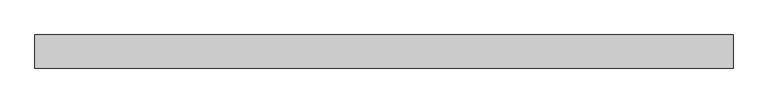
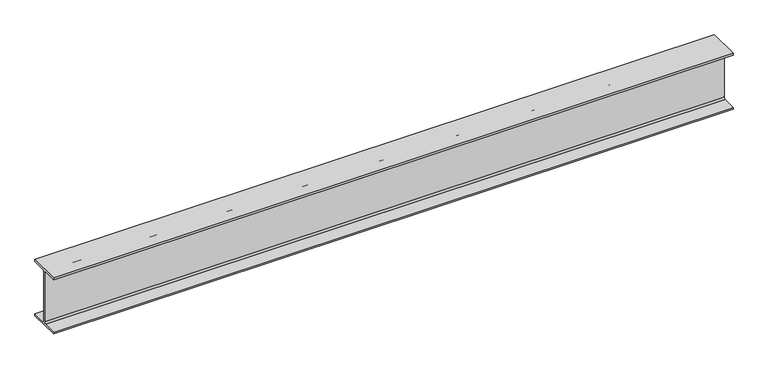
"""IFC4 building model written with IfcOpenShell, lengths in millimetres: beam geometry, Steel Beam_H-KSD3502 : H_SB_ASB_H-200x200x8x12."""

from ifc_helpers import new_model, si_unit, point, frame, frame_2d, origin, place, context, project, spatial, polyline, circle_curve, trimmed, segment, composite_curve, outline, extrude, source, transform, mapped, element, save


def beam_ba096bdf(model_context):
    return source(origin(), model_context, "Body", "SweptSolid", [
        extrude(outline(composite_curve([segment(polyline([(-82.5, -141.5), (-11.9, -141.5)]), True, "CONTINUOUS"), segment(trimmed(circle_curve(frame_2d((-11.9, -132.6)), 8.9), [point((-11.9, -141.5))], [point((-3.0, -132.6))], True, "CARTESIAN"), True, "CONTINUOUS"), segment(polyline([(-3.0, -132.6), (-3.0, 132.6)]), True, "CONTINUOUS"), segment(trimmed(circle_curve(frame_2d((-11.9, 132.6)), 8.9), [point((-3.0, 132.6))], [point((-11.9, 141.5))], True, "CARTESIAN"), True, "CONTINUOUS"), segment(polyline([(-11.9, 141.5), (-82.5, 141.5), (-82.5, 151.7), (82.5, 151.7), (82.5, 141.5), (11.9, 141.5)]), True, "CONTINUOUS"), segment(trimmed(circle_curve(frame_2d((11.9, 132.6)), 8.9), [point((11.9, 141.5))], [point((3.0, 132.6))], True, "CARTESIAN"), True, "CONTINUOUS"), segment(polyline([(3.0, 132.6), (3.0, -132.6)]), True, "CONTINUOUS"), segment(trimmed(circle_curve(frame_2d((11.9, -132.6)), 8.9), [point((3.0, -132.6))], [point((11.9, -141.5))], True, "CARTESIAN"), True, "CONTINUOUS"), segment(polyline([(11.9, -141.5), (82.5, -141.5), (82.5, -151.7), (-82.5, -151.7), (-82.5, -141.5)]), True, "CONTINUOUS")], self_intersect=False)), frame((-1756.1912669, 0.0, 0.0), z_axis=(1.0, 0.0, 0.0), x_axis=(0.0, 1.0, 0.0)), (0.0, 0.0, 1.0), 3479.0025034),
    ])


if __name__ == "__main__":
    model = new_model("IFC4")
    model_context = context("Model", 3, world=origin())
    ifc_project = project(units=[si_unit("LENGTHUNIT", "METRE", prefix="MILLI")], contexts=[model_context])
    site = spatial("IfcSite", under=ifc_project)
    building = spatial("IfcBuilding", under=site)
    placement = place(None, origin())
    beam_shape = beam_ba096bdf(model_context)
    element("IfcBeam", 1, ObjectType="Steel Beam_H-KSD3502 : H_SB_ASB_H-200x200x8x12", at=placement, inside=building, context=model_context, shape_type="MappedRepresentation", body=[
        mapped(beam_shape, transform((0.0, 0.0, 0.0), x_axis=(1.0, 0.0, 0.0), y_axis=(0.0, 1.0, 0.0), z_axis=(0.0, 0.0, 1.0))),
    ])
    save(model, "model.ifc")

# Revit data of these elements
# Type "Steel Beam_H-KSD3502 : H_SB_ASB_H-200x200x8x12"
#   Width = 20.0 cm
#   Web Thickness = 0.8 cm
#   Web Fillet = 1.3 cm
#   Warping Constant = 141376.0 cm⁶
#   Torsional Moment of Inertia = 26.2485 cm⁴
#   Torsional Modulus = 1.0 cm³
#   Section Area = 63.53 cm²
#   Plastic Modulus weak axis = 244.0 cm³
#   Plastic Modulus strong axis = 525.0 cm³
#   Perimeter = 1.16 m²/m
#   Nominal Weight = 49.90 kgf/m
#   Moment of Inertia weak axis = 1600.00 cm⁴
#   Moment of Inertia strong axis = 4720.00 cm⁴
#   Height = 20.0 cm
#   Flange Thickness = 1.2 cm
#   Elastic Modulus weak axis = 160.0 cm³
#   Elastic Modulus strong axis = 472.0 cm³
#   Centroid Vertical = 10.0 cm
#   Centroid Horizontal = 10.0 cm
#   Length [instance default] = 1.5240 m
#   Structural Material [instance default] = Steel, 45-345
#   Assembly Code = ""
# Element 1 (IfcBeam, "Steel Beam_H-KSD3502 : H_SB_ASB_H-200x200x8x12")
#   Structural Material = none
# Materials
#   "Steel, 45-345": class "Metal", colour RGB 189 187 185, transparency 0, Description = "Steel 345 MPa", Cost = 0
